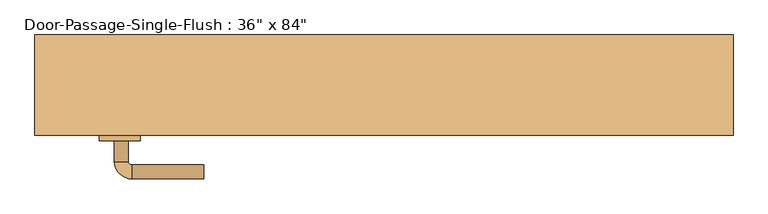
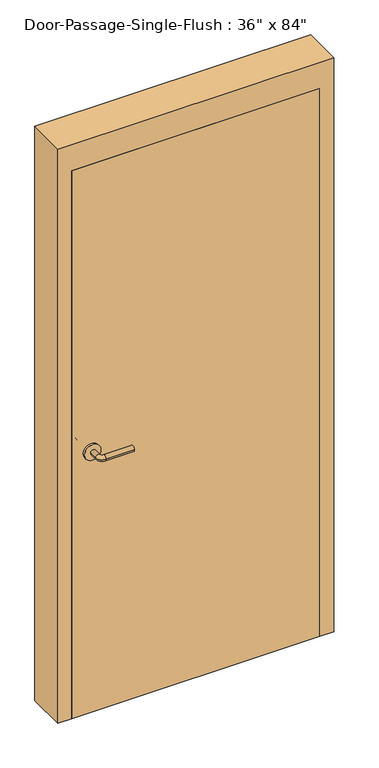
"""IFC4 building model written with IfcOpenShell, lengths in millimetres: door geometry."""

import ifcopenshell
import ifcopenshell.guid

model = None  # the IFC model being written
_history = None  # IfcOwnerHistory: only IFC2X3 demands one
_inside = {}  # id of a spatial element -> (the spatial element, [elements in it])
_under = {}  # id of a project, library or spatial element -> (it, [spatial elements below it])
_declared = {}  # id of a project -> (the project, [libraries it declares])
_typed = {}  # id of a type object -> (the type object, [elements of that type])
_made_of = {}  # id of a material, layer set ... -> (it, [elements and type objects made of it])


def new_model(schema):
    """Start an empty IFC model of exactly this schema.

    Asked for "IFC4X3", IfcOpenShell would pick the latest addendum, in which some entities
    have other attributes; the version numbers below select the first issue.
    IFC2X3 requires an IfcOwnerHistory on every rooted entity: one is made here for all.
    """
    global model, _history
    if schema == "IFC4X3":
        model = ifcopenshell.file(schema_version=(4, 3, 0, 0))
    else:
        model = ifcopenshell.file(schema=schema)
    _inside.clear()
    _under.clear()
    _declared.clear()
    _typed.clear()
    _made_of.clear()
    _history = None
    if model.schema == "IFC2X3":
        org = make("IfcOrganization", Name="unknown")
        user = make(
            "IfcPersonAndOrganization",
            ThePerson=make("IfcPerson", FamilyName="unknown"),
            TheOrganization=org,
        )
        app = make(
            "IfcApplication",
            ApplicationDeveloper=org,
            Version="unknown",
            ApplicationFullName="unknown",
            ApplicationIdentifier="unknown",
        )
        _history = make(
            "IfcOwnerHistory",
            OwningUser=user,
            OwningApplication=app,
            ChangeAction="ADDED",
            CreationDate=0,
        )
    return model


def make(cls, **values):
    """One entity of the class cls with the attributes given. An attribute that is None is left unset."""
    return model.create_entity(
        cls, **{name: value for name, value in values.items() if value is not None}
    )


def rooted(cls, **values):
    """An entity with a GlobalId (a new one), such as an element, a storey or a relation."""
    return make(cls, GlobalId=ifcopenshell.guid.new(), OwnerHistory=_history, **values)


def si_unit(unit_type, name, prefix=None):
    """IfcSIUnit, for example si_unit("LENGTHUNIT", "METRE", prefix="MILLI")."""
    return make("IfcSIUnit", UnitType=unit_type, Prefix=prefix, Name=name)


def assignment(units):
    """IfcUnitAssignment: the units of a project."""
    return None if units is None else make("IfcUnitAssignment", Units=units)


def point(xyz):
    """IfcCartesianPoint."""
    return None if xyz is None else make("IfcCartesianPoint", Coordinates=xyz)


def direction(xyz):
    """IfcDirection."""
    return None if xyz is None else make("IfcDirection", DirectionRatios=xyz)


def frame(location, z_axis=None, x_axis=None):
    """IfcAxis2Placement3D, a coordinate frame: its origin and axes. An axis left out is left unset."""
    return make(
        "IfcAxis2Placement3D",
        Location=point(location),
        Axis=direction(z_axis),
        RefDirection=direction(x_axis),
    )


def frame_2d(location, x_axis=None):
    """IfcAxis2Placement2D, a coordinate frame in the plane: its origin and x axis."""
    return make(
        "IfcAxis2Placement2D", Location=point(location), RefDirection=direction(x_axis)
    )


def origin():
    """The frame at (0, 0, 0) with its axes left unset."""
    return frame((0.0, 0.0, 0.0))


def origin_with_axes():
    """The frame at (0, 0, 0) with the z axis (0, 0, 1) and the x axis (1, 0, 0) written out."""
    return frame((0.0, 0.0, 0.0), z_axis=(0.0, 0.0, 1.0), x_axis=(1.0, 0.0, 0.0))


def place(relative_to, where):
    """IfcLocalPlacement: puts the frame where relative to a parent placement (None: the world)."""
    return make(
        "IfcLocalPlacement", PlacementRelTo=relative_to, RelativePlacement=where
    )


def context(
    kind, dimensions, precision=None, world=None, true_north=None, identifier=None
):
    """IfcGeometricRepresentationContext, for example the 3D "Model" context."""
    return make(
        "IfcGeometricRepresentationContext",
        ContextIdentifier=identifier,
        ContextType=kind,
        CoordinateSpaceDimension=dimensions,
        Precision=precision,
        WorldCoordinateSystem=world,
        TrueNorth=true_north,
    )


def project(units=None, contexts=None):
    """IfcProject with its units and contexts."""
    return rooted(
        "IfcProject",
        Name="project",
        RepresentationContexts=contexts,
        UnitsInContext=assignment(units),
    )


def spatial(cls, under=None, at=None, **own):
    """A site, building, storey or space (cls), placed at a placement, below another one or the project."""
    s = rooted(cls, ObjectPlacement=at, **own)
    if under is not None:
        _under.setdefault(under.id(), (under, []))[1].append(s)
    return s


def polyline(points):
    """IfcPolyline through the points."""
    return make("IfcPolyline", Points=[point(p) for p in points])


def circle_curve(where, radius):
    """IfcCircle in the frame where."""
    return make("IfcCircle", Position=where, Radius=radius)


def ellipse_curve(where, semi_axis1, semi_axis2):
    """IfcEllipse in the frame where."""
    return make(
        "IfcEllipse", Position=where, SemiAxis1=semi_axis1, SemiAxis2=semi_axis2
    )


def trimmed(basis, trim1, trim2, sense, master):
    """IfcTrimmedCurve: the piece of a basis curve between two trims."""
    return make(
        "IfcTrimmedCurve",
        BasisCurve=basis,
        Trim1=trim1,
        Trim2=trim2,
        SenseAgreement=sense,
        MasterRepresentation=master,
    )


def segment(curve, same_sense, transition):
    """IfcCompositeCurveSegment."""
    return make(
        "IfcCompositeCurveSegment",
        Transition=transition,
        SameSense=same_sense,
        ParentCurve=curve,
    )


def composite_curve(segments, self_intersect=None):
    """IfcCompositeCurve: segments joined end to end."""
    return make("IfcCompositeCurve", Segments=segments, SelfIntersect=self_intersect)


def outline(outer, holes=None, kind="AREA"):
    """IfcArbitraryClosedProfileDef: a profile drawn as a closed curve; with holes, ...WithVoids."""
    if holes is None:
        return make("IfcArbitraryClosedProfileDef", ProfileType=kind, OuterCurve=outer)
    return make(
        "IfcArbitraryProfileDefWithVoids",
        ProfileType=kind,
        OuterCurve=outer,
        InnerCurves=holes,
    )


def extrude(swept, where, along, depth):
    """IfcExtrudedAreaSolid: the profile swept, set in the frame where, extruded along a direction by depth."""
    return make(
        "IfcExtrudedAreaSolid",
        SweptArea=swept,
        Position=where,
        ExtrudedDirection=direction(along),
        Depth=depth,
    )


def faces_of(points, faces, orient=None, outer=None):
    """IfcFace entities. A face is a list of loops; a loop is a list of indices into points, from 0.

    orient and outer hold one flag for each loop. By default every Orientation is true, the
    first loop of a face is its IfcFaceOuterBound and the others are IfcFaceBound.
    """
    made = []
    for i, loops in enumerate(faces):
        bounds = []
        for j, loop in enumerate(loops):
            is_outer = j == 0 if outer is None else outer[i][j]
            bounds.append(
                make(
                    "IfcFaceOuterBound" if is_outer else "IfcFaceBound",
                    Bound=make("IfcPolyLoop", Polygon=[points[k] for k in loop]),
                    Orientation=True if orient is None else orient[i][j],
                )
            )
        made.append(make("IfcFace", Bounds=bounds))
    return made


def faceted_brep(points, faces, orient=None, outer=None, voids=None):
    """IfcFacetedBrep: a solid bounded by flat faces; with voids (closed shells), ...WithVoids."""
    shared = [point(p) for p in points]
    hull = make("IfcClosedShell", CfsFaces=faces_of(shared, faces, orient, outer))
    if voids is None:
        return make("IfcFacetedBrep", Outer=hull)
    return make(
        "IfcFacetedBrepWithVoids",
        Outer=hull,
        Voids=[
            make(cls, CfsFaces=faces_of(shared, fs, o, b)) for cls, fs, o, b in voids
        ],
    )


def shape(context_of_items, identifier, shape_type, items):
    """IfcShapeRepresentation: the items that make up one representation, for example the "Body"."""
    return make(
        "IfcShapeRepresentation",
        ContextOfItems=context_of_items,
        RepresentationIdentifier=identifier,
        RepresentationType=shape_type,
        Items=items,
    )


def source(mapping_origin, context_of_items, identifier, shape_type, items):
    """IfcRepresentationMap: a shape defined once, which mapped items show again and again."""
    return make(
        "IfcRepresentationMap",
        MappingOrigin=mapping_origin,
        MappedRepresentation=shape(context_of_items, identifier, shape_type, items),
    )


def transform(
    local_origin,
    x_axis=None,
    y_axis=None,
    z_axis=None,
    scale=None,
    scale2=None,
    scale3=None,
    uniform=True,
):
    """IfcCartesianTransformationOperator3D, or its non-uniform kind. x_axis, y_axis, z_axis: its Axis1, 2, 3."""
    if uniform:
        return make(
            "IfcCartesianTransformationOperator3D",
            Axis1=direction(x_axis),
            Axis2=direction(y_axis),
            LocalOrigin=point(local_origin),
            Scale=scale,
            Axis3=direction(z_axis),
        )
    return make(
        "IfcCartesianTransformationOperator3DnonUniform",
        Axis1=direction(x_axis),
        Axis2=direction(y_axis),
        LocalOrigin=point(local_origin),
        Scale=scale,
        Axis3=direction(z_axis),
        Scale2=scale2,
        Scale3=scale3,
    )


def mapped(mapping_source, mapping_target):
    """IfcMappedItem: shows the shape of a source again, moved by a transform."""
    return make(
        "IfcMappedItem", MappingSource=mapping_source, MappingTarget=mapping_target
    )


def made_of(thing, what):
    """Note that an element or type object is made of a material, layer set ...; save() writes the relation."""
    if what is not None:
        _made_of.setdefault(what.id(), (what, []))[1].append(thing)
    return thing


def element(
    cls,
    number,
    at=None,
    inside=None,
    cuts=None,
    type_object=None,
    material=None,
    context=None,
    identifier="Body",
    shape_type=None,
    held_by="IfcProductDefinitionShape",
    body=None,
    shapes=None,
    **own,
):
    """One element of the class cls, such as IfcWall. Its Tag is "e" and its number.

    at: its placement. inside: the storey or other place that contains it. cuts: it is an
    opening in that element (IfcRelVoidsElement). A single representation is given by context,
    identifier, shape_type and body (its items); several are given by shapes. held_by: the class
    of the entity that holds the representations. save() writes the other relations.
    """
    e = rooted(cls, Tag="e%d" % number, ObjectPlacement=at, **own)
    if body is not None:
        shapes = [shape(context, identifier, shape_type, body)]
    if shapes is not None:
        e.Representation = make(held_by, Representations=shapes)
    if inside is not None:
        _inside.setdefault(inside.id(), (inside, []))[1].append(e)
    if cuts is not None:
        rooted(
            "IfcRelVoidsElement", RelatingBuildingElement=cuts, RelatedOpeningElement=e
        )
    if type_object is not None:
        _typed.setdefault(type_object.id(), (type_object, []))[1].append(e)
    return made_of(e, material)


def aggregate(whole, parts):
    """IfcRelAggregates: a whole, such as a stair, and the parts it consists of."""
    return rooted("IfcRelAggregates", RelatingObject=whole, RelatedObjects=parts)


def save(model, path):
    """Write the relations noted so far, then the file.

    IfcRelAggregates (storeys below a building ...), IfcRelContainedInSpatialStructure (elements
    in a storey), IfcRelDefinesByType, IfcRelAssociatesMaterial and IfcRelDeclares: one each for
    every whole, place, type object, material and project.
    """
    for whole, parts in _under.values():
        aggregate(whole, parts)
    for where, things in _inside.values():
        rooted(
            "IfcRelContainedInSpatialStructure",
            RelatedElements=things,
            RelatingStructure=where,
        )
    for kind, things in _typed.values():
        rooted("IfcRelDefinesByType", RelatedObjects=things, RelatingType=kind)
    for what, things in _made_of.values():
        rooted("IfcRelAssociatesMaterial", RelatedObjects=things, RelatingMaterial=what)
    for by, libraries in _declared.values():
        rooted("IfcRelDeclares", RelatingContext=by, RelatedDefinitions=libraries)
    model.write(path)


def plane_surface(at):
    """IfcPlane: the flat surface through the origin of the frame at, square to its z axis."""
    return make("IfcPlane", Position=at)


def cylinder_surface(at, radius):
    """IfcCylindricalSurface: all points at the distance radius from the z axis of the frame at."""
    return make("IfcCylindricalSurface", Position=at, Radius=radius)


def revolved_surface(curve, axis_point, axis_direction):
    """IfcSurfaceOfRevolution: the curve turned about the line through axis_point along axis_direction."""
    return make(
        "IfcSurfaceOfRevolution",
        SweptCurve=make("IfcArbitraryOpenProfileDef", ProfileType="CURVE", Curve=curve),
        AxisPosition=make("IfcAxis1Placement", Location=point(axis_point), Axis=direction(axis_direction)),
    )


def advanced_brep(points, edges, surfaces, faces):
    """IfcAdvancedBrep: a solid bounded by faces that lie on surfaces and meet in shared edges.

    An edge is (start, end): straight between two places in points (the first is 0);
    or (start, end, curve); or (start, end, curve, False) where it runs against its curve.
    A face is (place in surfaces, loops), or (place, loops, False) where it looks against
    its surface's normal. A loop lists edges by number (the first is 1), with a minus sign
    where the edge is run from its end to its start. The first loop is the outer one.
    """
    corners = [point(p) for p in points]
    vertices = [make("IfcVertexPoint", VertexGeometry=c) for c in corners]
    made = []
    for start, end, *more in edges:
        made.append(
            make(
                "IfcEdgeCurve",
                EdgeStart=vertices[start],
                EdgeEnd=vertices[end],
                EdgeGeometry=more[0] if more else make("IfcPolyline", Points=[corners[start], corners[end]]),
                SameSense=more[1] if len(more) > 1 else True,
            )
        )
    hull = []
    for where, loops, *sense in faces:
        bounds = []
        for j, loop in enumerate(loops):
            ring = [make("IfcOrientedEdge", EdgeElement=made[abs(k) - 1], Orientation=k > 0) for k in loop]
            bounds.append(
                make(
                    "IfcFaceOuterBound" if j == 0 else "IfcFaceBound",
                    Bound=make("IfcEdgeLoop", EdgeList=ring),
                    Orientation=True,
                )
            )
        hull.append(make("IfcAdvancedFace", Bounds=bounds, FaceSurface=surfaces[where], SameSense=sense[0] if sense else True))
    return make("IfcAdvancedBrep", Outer=make("IfcClosedShell", CfsFaces=hull))


def door_9f6fe377(model_context):
    return source(origin(), model_context, "Body", "SolidModel", [
        advanced_brep(
        [(-392.190625, -25.3375, 1016.0), (-372.190625, -25.3375, 1016.0), (-392.190625, 4.6625, 1016.0), (-372.190625, 4.6625, 1016.0), (-367.190625, 9.6625, 1016.0), (-367.190625, 29.6625, 1016.0), (-262.190625, 29.6625, 1016.0), (-262.190625, 9.6625, 1016.0)],
        [
            (0, 1, circle_curve(frame((-382.190625, -25.3375, 1016.0), z_axis=(0.0, -1.0, 0.0), x_axis=(1.0, 0.0, 0.0)), 10.0)),
            (1, 0, circle_curve(frame((-382.190625, -25.3375, 1016.0), z_axis=(0.0, -1.0, 0.0), x_axis=(1.0, 0.0, 0.0)), 10.0)),
            (0, 2),
            (2, 3, circle_curve(frame((-382.190625, 4.6625, 1016.0), z_axis=(0.0, -1.0, 0.0), x_axis=(1.0, 0.0, 0.0)), 10.0)),
            (3, 1),
            (3, 2, circle_curve(frame((-382.190625, 4.6625, 1016.0), z_axis=(0.0, -1.0, 0.0), x_axis=(1.0, 0.0, 0.0)), 10.0)),
            (4, 3, circle_curve(frame((-367.190625, 4.6625, 1016.0), z_axis=(0.0, 0.0, 1.0), x_axis=(-1.0, 0.0, 0.0)), 5.0)),
            (2, 5, circle_curve(frame((-367.190625, 4.6625, 1016.0), z_axis=(0.0, 0.0, -1.0), x_axis=(-1.0, 0.0, 0.0)), 25.0)),
            (5, 4, circle_curve(frame((-367.190625, 19.6625, 1016.0), z_axis=(-1.0, 0.0, 0.0), x_axis=(0.0, -1.0, 0.0)), 10.0)),
            (4, 5, circle_curve(frame((-367.190625, 19.6625, 1016.0), z_axis=(-1.0, 0.0, 0.0), x_axis=(0.0, -1.0, 0.0)), 10.0)),
            (6, 7, circle_curve(frame((-262.190625, 19.6625, 1016.0), z_axis=(1.0, 0.0, 0.0), x_axis=(0.0, -1.0, 0.0)), 10.0)),
            (7, 6, circle_curve(frame((-262.190625, 19.6625, 1016.0), z_axis=(1.0, 0.0, 0.0), x_axis=(0.0, -1.0, 0.0)), 10.0)),
            (5, 6),
            (7, 4),
        ],
        [
            plane_surface(frame((-382.190625, -25.3375, 1016.0), z_axis=(0.0, -1.0, 0.0), x_axis=(0.0, 0.0, 1.0))),
            cylinder_surface(frame((-382.190625, -25.3375, 1016.0), z_axis=(0.0, -1.0, 0.0), x_axis=(1.0, 0.0, 0.0)), 10.0),
            revolved_surface(trimmed(ellipse_curve(frame((-382.190625, 4.6625, 1016.0), z_axis=(0.0, -1.0, 0.0), x_axis=(1.0, 0.0, 0.0)), 10.0, 10.0), [point((-392.190625, 4.6625, 1016.0))], [point((-372.190625, 4.6625, 1016.0))], True, "CARTESIAN"), (-367.190625, 4.6625, 1016.0), (0.0, 0.0, -1.0)),
            revolved_surface(trimmed(ellipse_curve(frame((-382.190625, 4.6625, 1016.0), z_axis=(0.0, -1.0, 0.0), x_axis=(1.0, 0.0, 0.0)), 10.0, 10.0), [point((-372.190625, 4.6625, 1016.0))], [point((-392.190625, 4.6625, 1016.0))], True, "CARTESIAN"), (-367.190625, 4.6625, 1016.0), (0.0, 0.0, -1.0)),
            plane_surface(frame((-262.190625, 19.6625, 1016.0), z_axis=(1.0, 0.0, 0.0), x_axis=(0.0, 0.0, 1.0))),
            cylinder_surface(frame((-367.190625, 19.6625, 1016.0), z_axis=(-1.0, 0.0, 0.0), x_axis=(0.0, -1.0, 0.0)), 10.0),
        ],
        [
            (0, [[1, 2]]),
            (1, [[-1, 3, 4, 5]]),
            (1, [[-2, -5, 6, -3]]),
            (2, [[7, -4, 8, 9]]),
            (3, [[-8, -6, -7, 10]]),
            (4, [[11, 12]]),
            (5, [[-9, 13, -12, 14]]),
            (5, [[-10, -14, -11, -13]]),
        ],
    ),
        extrude(outline(composite_curve([segment(trimmed(circle_curve(frame_2d((1016.0, -384.690625)), 30.0), [point((1016.0, -414.690625))], [point((1016.0, -354.690625))], False, "CARTESIAN"), True, "CONTINUOUS"), segment(trimmed(circle_curve(frame_2d((1016.0, -384.690625)), 30.0), [point((1016.0, -354.690625))], [point((1016.0, -414.690625))], False, "CARTESIAN"), True, "CONTINUOUS")], self_intersect=False)), frame((0.0, -33.3375, 0.0), z_axis=(0.0, 1.0, 0.0), x_axis=(0.0, 0.0, 1.0)), (0.0, 0.0, 1.0), 8.0),
        advanced_brep(
        [(-392.190625, -85.7875, 1016.0), (-372.190625, -85.7875, 1016.0), (-372.190625, -115.7875, 1016.0), (-392.190625, -115.7875, 1016.0), (-367.190625, -120.7875, 1016.0), (-367.190625, -140.7875, 1016.0), (-262.190625, -140.7875, 1016.0), (-262.190625, -120.7875, 1016.0)],
        [
            (0, 1, circle_curve(frame((-382.190625, -85.7875, 1016.0), z_axis=(0.0, 1.0, 0.0), x_axis=(1.0, 0.0, 0.0)), 10.0)),
            (1, 0, circle_curve(frame((-382.190625, -85.7875, 1016.0), z_axis=(0.0, 1.0, 0.0), x_axis=(1.0, 0.0, 0.0)), 10.0)),
            (1, 2),
            (2, 3, circle_curve(frame((-382.190625, -115.7875, 1016.0), z_axis=(0.0, 1.0, 0.0), x_axis=(1.0, 0.0, 0.0)), 10.0)),
            (3, 0),
            (3, 2, circle_curve(frame((-382.190625, -115.7875, 1016.0), z_axis=(0.0, 1.0, 0.0), x_axis=(1.0, 0.0, 0.0)), 10.0)),
            (4, 5, circle_curve(frame((-367.190625, -130.7875, 1016.0), z_axis=(-1.0, 0.0, 0.0), x_axis=(0.0, 1.0, 0.0)), 10.0)),
            (5, 3, circle_curve(frame((-367.190625, -115.7875, 1016.0), z_axis=(0.0, 0.0, -1.0), x_axis=(-1.0, 0.0, 0.0)), 25.0)),
            (2, 4, circle_curve(frame((-367.190625, -115.7875, 1016.0), z_axis=(0.0, 0.0, 1.0), x_axis=(-1.0, 0.0, 0.0)), 5.0)),
            (5, 4, circle_curve(frame((-367.190625, -130.7875, 1016.0), z_axis=(-1.0, 0.0, 0.0), x_axis=(0.0, 1.0, 0.0)), 10.0)),
            (6, 7, circle_curve(frame((-262.190625, -130.7875, 1016.0), z_axis=(1.0, 0.0, 0.0), x_axis=(0.0, 1.0, 0.0)), 10.0)),
            (7, 6, circle_curve(frame((-262.190625, -130.7875, 1016.0), z_axis=(1.0, 0.0, 0.0), x_axis=(0.0, 1.0, 0.0)), 10.0)),
            (4, 7),
            (6, 5),
        ],
        [
            plane_surface(frame((-382.190625, -85.7875, 1016.0), z_axis=(0.0, 1.0, 0.0), x_axis=(0.0, 0.0, 1.0))),
            cylinder_surface(frame((-382.190625, -85.7875, 1016.0), z_axis=(0.0, 1.0, 0.0), x_axis=(1.0, 0.0, 0.0)), 10.0),
            revolved_surface(trimmed(ellipse_curve(frame((-382.190625, -115.7875, 1016.0), z_axis=(0.0, -1.0, 0.0), x_axis=(1.0, 0.0, 0.0)), 10.0, 10.0), [point((-392.190625, -115.7875, 1016.0))], [point((-372.190625, -115.7875, 1016.0))], True, "CARTESIAN"), (-367.190625, -115.7875, 1016.0), (0.0, 0.0, -1.0)),
            revolved_surface(trimmed(ellipse_curve(frame((-382.190625, -115.7875, 1016.0), z_axis=(0.0, -1.0, 0.0), x_axis=(1.0, 0.0, 0.0)), 10.0, 10.0), [point((-372.190625, -115.7875, 1016.0))], [point((-392.190625, -115.7875, 1016.0))], True, "CARTESIAN"), (-367.190625, -115.7875, 1016.0), (0.0, 0.0, -1.0)),
            plane_surface(frame((-262.190625, -130.7875, 1016.0), z_axis=(1.0, 0.0, 0.0), x_axis=(0.0, 0.0, 1.0))),
            cylinder_surface(frame((-367.190625, -130.7875, 1016.0), z_axis=(-1.0, 0.0, 0.0), x_axis=(0.0, 1.0, 0.0)), 10.0),
        ],
        [
            (0, [[1, 2]]),
            (1, [[3, 4, 5, -2]]),
            (1, [[-5, 6, -3, -1]]),
            (2, [[7, 8, -4, 9]]),
            (3, [[10, -9, -6, -8]]),
            (4, [[11, 12]]),
            (5, [[13, -11, 14, -7]]),
            (5, [[-14, -12, -13, -10]]),
        ],
    ),
        extrude(outline(composite_curve([segment(trimmed(circle_curve(frame_2d((1016.0, -384.690625)), 30.0), [point((1016.0, -414.690625))], [point((1016.0, -354.690625))], False, "CARTESIAN"), True, "CONTINUOUS"), segment(trimmed(circle_curve(frame_2d((1016.0, -384.690625)), 30.0), [point((1016.0, -354.690625))], [point((1016.0, -414.690625))], False, "CARTESIAN"), True, "CONTINUOUS")], self_intersect=False)), frame((0.0, -85.7875, 0.0), z_axis=(0.0, 1.0, 0.0), x_axis=(0.0, 0.0, 1.0)), (0.0, 0.0, 1.0), 8.0),
        faceted_brep([(457.2, -28.575, 0.0), (441.325, -28.575, 0.0), (441.325, 19.05, 0.0), (457.2, 19.05, 0.0), (457.2, 68.2625, 0.0), (508.0, 68.2625, 0.0), (508.0, -77.7875, 0.0), (457.2, -77.7875, 0.0), (457.2, -77.7875, 2133.6), (457.2, -28.575, 2133.6), (508.0, -77.7875, 2235.2), (-508.0, -77.7875, 2235.2), (-508.0, -77.7875, 0.0), (-457.2, -77.7875, 0.0), (-457.2, -77.7875, 2133.6), (508.0, 68.2625, 2235.2), (457.2, 68.2625, 2133.6), (-457.2, 68.2625, 2133.6), (-457.2, 68.2625, 0.0), (-508.0, 68.2625, 0.0), (-508.0, 68.2625, 2235.2), (457.2, 19.05, 2133.6), (441.325, 19.05, 2117.725), (-441.325, 19.05, 2117.725), (-441.325, 19.05, 0.0), (-457.2, 19.05, 0.0), (-457.2, 19.05, 2133.6), (441.325, -28.575, 2117.725), (-457.2, -28.575, 2133.6), (-457.2, -28.575, 0.0), (-441.325, -28.575, 0.0), (-441.325, -28.575, 2117.725)], [[[0, 1, 2, 3, 4, 5, 6, 7]], [[7, 8, 9, 0]], [[6, 10, 11, 12, 13, 14, 8, 7]], [[5, 15, 10, 6]], [[4, 16, 17, 18, 19, 20, 15, 5]], [[3, 21, 16, 4]], [[2, 22, 23, 24, 25, 26, 21, 3]], [[1, 27, 22, 2]], [[0, 9, 28, 29, 30, 31, 27, 1]], [[8, 14, 28, 9]], [[16, 21, 26, 17]], [[22, 27, 31, 23]], [[12, 19, 18, 25, 24, 30, 29, 13]], [[13, 29, 28, 14]], [[11, 20, 19, 12]], [[17, 26, 25, 18]], [[23, 31, 30, 24]], [[15, 20, 11, 10]]]),
        extrude(outline(polyline([(457.2, -33.3375), (457.2, -77.7875), (-457.2, -77.7875), (-457.2, -33.3375), (457.2, -33.3375)])), origin_with_axes(), (0.0, 0.0, 1.0), 2133.6),
    ])


if __name__ == "__main__":
    model = new_model("IFC4")
    model_context = context("Model", 3, world=origin())
    ifc_project = project(units=[si_unit("LENGTHUNIT", "METRE", prefix="MILLI")], contexts=[model_context])
    site = spatial("IfcSite", under=ifc_project)
    building = spatial("IfcBuilding", under=site)
    placement = place(None, origin())
    door_shape = door_9f6fe377(model_context)
    element("IfcDoor", 1, ObjectType="Door-Passage-Single-Flush : 36\" x 84\"", at=placement, inside=building, context=model_context, shape_type="MappedRepresentation", body=[
        mapped(door_shape, transform((0.0, 0.0, 0.0), x_axis=(1.0, 0.0, 0.0), y_axis=(0.0, 1.0, 0.0), z_axis=(0.0, 0.0, 1.0))),
    ])
    save(model, "model.ifc")

# Revit data of these elements
# Type "Door-Passage-Single-Flush : 36\" x 84\""
#   Type Mark = "1"
#   Assembly Code = "B2030200"
#   Analytic Construction = "Wooden"
#   Thickness = 0' - 1 3/4"
#   Thermal Resistance (R) = 2.5876 (h·ft²·°F)/BTU
#   Swing Angle [instance default] = 90.00°
#   Strike Height = 3' - 4"
#   Rough Width [instance default] = 3' - 4"
#   Rough Height [instance default] = 7' - 4"
#   MF Opening Height [instance default] = 0' - 4"
#   MF Opening Width [instance default] = 0' - 4"
#   Inset Calculate [instance default] = 0' - 4"
#   Masonry Inset [instance default] = 0' - 1"
#   Height = 7' - 0"
#   Width = 3' - 0"
#   Heat Transfer Coefficient (U) = 0.3865 BTU/(h·ft²·°F)
#   Masonry Frame Depth = 0' - 5 3/4"
#   Define Thermal Properties by = 1
#   Masonry Frame [instance default] = yes
#   Function = 1
#   Dry Wall Frame [instance default] = no
#   Panel Material = Wood - Birch
#   Frame Material = Metal - Paint Finish - Grey
#   Door Handle Material = Aluminum
#   Visual Light Transmittance = 0
#   Solar Heat Gain Coefficient = 0
#   Wall Closure = (empty or 0)
# Element 1 (IfcDoor, "Door-Passage-Single-Flush : 36\" x 84\"")
#   Materials on its faces: "Aluminum", "Metal - Paint Finish - Grey", "Wood - Birch"
# Materials
#   "Wood - Birch": class "Wood", colour RGB 166 116 52, transparency 0, Cost = 0
#   "Metal - Paint Finish - Grey": class "Paint", colour RGB 104 104 104, transparency 0, Cost = 0
#   "Aluminum": class "Metal", colour RGB 247 247 247, transparency 0, Description = "Aluminum 6061", Cost = 0
